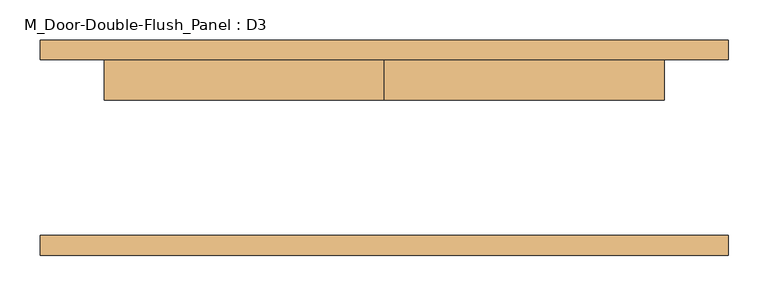
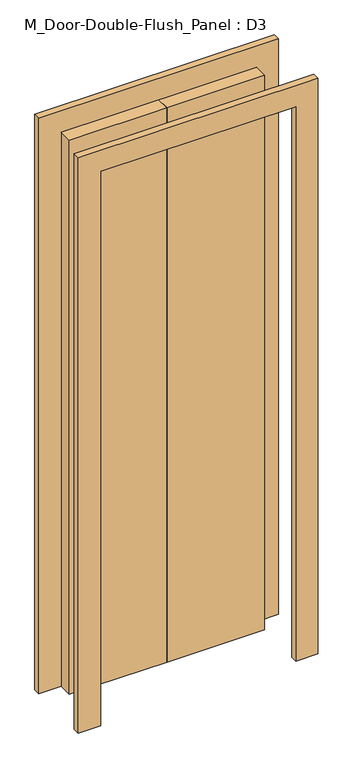
"""IFC4 building model written with IfcOpenShell, lengths in millimetres: door geometry, M_Door-Double-Flush_Panel : D3."""

from ifc_helpers import new_model, si_unit, frame, origin, origin_with_axes, place, context, project, spatial, polyline, outline, extrude, source, transform, mapped, element, save


def m_door_double_flush_panel_d3_82d72d24(model_context):
    return source(origin(), model_context, "Body", "SweptSolid", [
        extrude(outline(polyline([(2100.0, -350.0), (2100.0, 350.0), (0.0, 350.0), (0.0, 430.0), (2180.0, 430.0), (2180.0, -430.0), (0.0, -430.0), (0.0, -350.0), (2100.0, -350.0)])), frame((0.0, -135.0, 0.0), z_axis=(0.0, 1.0, 0.0), x_axis=(0.0, 0.0, 1.0)), (0.0, 0.0, 1.0), 25.0),
        extrude(outline(polyline([(2100.0, -350.0), (2100.0, 350.0), (0.0, 350.0), (0.0, 430.0), (2180.0, 430.0), (2180.0, -430.0), (0.0, -430.0), (0.0, -350.0), (2100.0, -350.0)])), frame((0.0, 110.0, 0.0), z_axis=(0.0, 1.0, 0.0), x_axis=(0.0, 0.0, 1.0)), (0.0, 0.0, 1.0), 25.0),
        extrude(outline(polyline([(0.0, 110.0), (350.0, 110.0), (350.0, 60.0), (0.0, 60.0), (0.0, 110.0)])), origin_with_axes(), (0.0, 0.0, 1.0), 2100.0),
        extrude(outline(polyline([(-350.0, 110.0), (0.0, 110.0), (0.0, 60.0), (-350.0, 60.0), (-350.0, 110.0)])), origin_with_axes(), (0.0, 0.0, 1.0), 2100.0),
    ])


if __name__ == "__main__":
    model = new_model("IFC4")
    model_context = context("Model", 3, world=origin())
    ifc_project = project(units=[si_unit("LENGTHUNIT", "METRE", prefix="MILLI")], contexts=[model_context])
    site = spatial("IfcSite", under=ifc_project)
    building = spatial("IfcBuilding", under=site)
    placement = place(None, origin())
    m_door_double_flush_panel_d3_shape = m_door_double_flush_panel_d3_82d72d24(model_context)
    element("IfcDoor", 1, ObjectType="M_Door-Double-Flush_Panel : D3", at=placement, inside=building, context=model_context, shape_type="MappedRepresentation", body=[
        mapped(m_door_double_flush_panel_d3_shape, transform((0.0, 0.0, 0.0), x_axis=(1.0, 0.0, 0.0), y_axis=(0.0, 1.0, 0.0), z_axis=(0.0, 0.0, 1.0))),
    ])
    save(model, "model.ifc")

# Revit data of these elements
# Type "M_Door-Double-Flush_Panel : D3"
#   Type Mark = "57"
#   Construction Type Id = "DOOR"
#   Assembly Code = "C1020"
#   Analytic Construction = "Wooden"
#   Thickness = 5 cm
#   Thermal Resistance (R) = 0.455703 (m²·K)/W
#   Swing Angle [instance default] = 90.00°
#   Panel Width = 35 cm
#   Heat Transfer Coefficient (U) = 2.19465 W/(m²·K)
#   Height = 210 cm
#   Trim Projection Ext = 2.5 cm
#   Trim Projection Int = 2.5 cm
#   Trim Width = 8 cm
#   Width = 70 cm
#   Panel Material = Wood - Birch - Solid Stained Light Low Gloss
#   Trim Material = Paint - Sienna
#   Visual Light Transmittance = 0
#   Solar Heat Gain Coefficient = 0
#   Function = (empty or 0)
#   Wall Closure = (empty or 0)
# Element 1 (IfcDoor, "M_Door-Double-Flush_Panel : D3")
#   Materials on its faces: "Paint - Sienna", "Wood - Birch - Solid Stained Light Low Gloss"
# Materials
#   "Wood - Birch - Solid Stained Light Low Gloss": class "Wood", colour RGB 210 159 95, transparency 0, Cost = 0
#   "Paint - Sienna": class "Miscellaneous", colour RGB 118 70 51, transparency 0, Cost = 0
